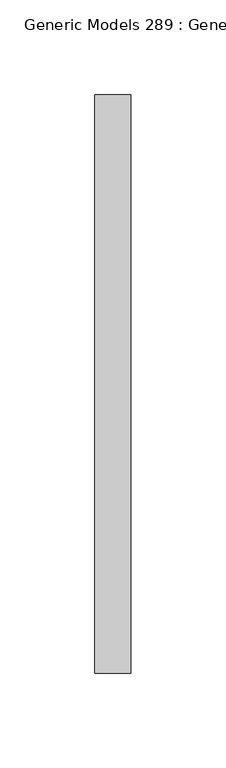
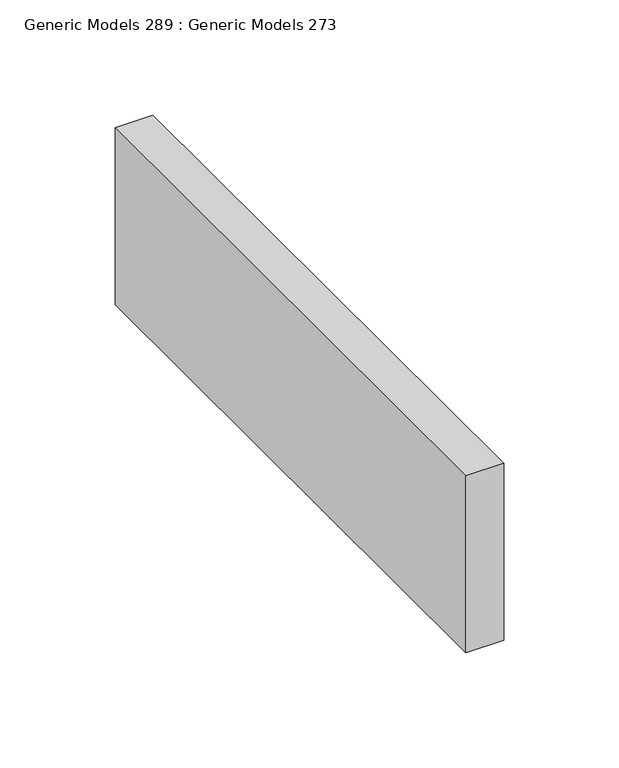
"""IFC4 building model written with IfcOpenShell, lengths in millimetres: proxy geometry, Generic Models 289 : Generic Models 273."""

import ifcopenshell
import ifcopenshell.guid

model = None  # the IFC model being written
_history = None  # IfcOwnerHistory: only IFC2X3 demands one
_inside = {}  # id of a spatial element -> (the spatial element, [elements in it])
_under = {}  # id of a project, library or spatial element -> (it, [spatial elements below it])
_declared = {}  # id of a project -> (the project, [libraries it declares])
_typed = {}  # id of a type object -> (the type object, [elements of that type])
_made_of = {}  # id of a material, layer set ... -> (it, [elements and type objects made of it])


def new_model(schema):
    """Start an empty IFC model of exactly this schema.

    Asked for "IFC4X3", IfcOpenShell would pick the latest addendum, in which some entities
    have other attributes; the version numbers below select the first issue.
    IFC2X3 requires an IfcOwnerHistory on every rooted entity: one is made here for all.
    """
    global model, _history
    if schema == "IFC4X3":
        model = ifcopenshell.file(schema_version=(4, 3, 0, 0))
    else:
        model = ifcopenshell.file(schema=schema)
    _inside.clear()
    _under.clear()
    _declared.clear()
    _typed.clear()
    _made_of.clear()
    _history = None
    if model.schema == "IFC2X3":
        org = make("IfcOrganization", Name="unknown")
        user = make(
            "IfcPersonAndOrganization",
            ThePerson=make("IfcPerson", FamilyName="unknown"),
            TheOrganization=org,
        )
        app = make(
            "IfcApplication",
            ApplicationDeveloper=org,
            Version="unknown",
            ApplicationFullName="unknown",
            ApplicationIdentifier="unknown",
        )
        _history = make(
            "IfcOwnerHistory",
            OwningUser=user,
            OwningApplication=app,
            ChangeAction="ADDED",
            CreationDate=0,
        )
    return model


def make(cls, **values):
    """One entity of the class cls with the attributes given. An attribute that is None is left unset."""
    return model.create_entity(
        cls, **{name: value for name, value in values.items() if value is not None}
    )


def rooted(cls, **values):
    """An entity with a GlobalId (a new one), such as an element, a storey or a relation."""
    return make(cls, GlobalId=ifcopenshell.guid.new(), OwnerHistory=_history, **values)


def si_unit(unit_type, name, prefix=None):
    """IfcSIUnit, for example si_unit("LENGTHUNIT", "METRE", prefix="MILLI")."""
    return make("IfcSIUnit", UnitType=unit_type, Prefix=prefix, Name=name)


def assignment(units):
    """IfcUnitAssignment: the units of a project."""
    return None if units is None else make("IfcUnitAssignment", Units=units)


def point(xyz):
    """IfcCartesianPoint."""
    return None if xyz is None else make("IfcCartesianPoint", Coordinates=xyz)


def direction(xyz):
    """IfcDirection."""
    return None if xyz is None else make("IfcDirection", DirectionRatios=xyz)


def frame(location, z_axis=None, x_axis=None):
    """IfcAxis2Placement3D, a coordinate frame: its origin and axes. An axis left out is left unset."""
    return make(
        "IfcAxis2Placement3D",
        Location=point(location),
        Axis=direction(z_axis),
        RefDirection=direction(x_axis),
    )


def origin():
    """The frame at (0, 0, 0) with its axes left unset."""
    return frame((0.0, 0.0, 0.0))


def place(relative_to, where):
    """IfcLocalPlacement: puts the frame where relative to a parent placement (None: the world)."""
    return make(
        "IfcLocalPlacement", PlacementRelTo=relative_to, RelativePlacement=where
    )


def context(
    kind, dimensions, precision=None, world=None, true_north=None, identifier=None
):
    """IfcGeometricRepresentationContext, for example the 3D "Model" context."""
    return make(
        "IfcGeometricRepresentationContext",
        ContextIdentifier=identifier,
        ContextType=kind,
        CoordinateSpaceDimension=dimensions,
        Precision=precision,
        WorldCoordinateSystem=world,
        TrueNorth=true_north,
    )


def project(units=None, contexts=None):
    """IfcProject with its units and contexts."""
    return rooted(
        "IfcProject",
        Name="project",
        RepresentationContexts=contexts,
        UnitsInContext=assignment(units),
    )


def spatial(cls, under=None, at=None, **own):
    """A site, building, storey or space (cls), placed at a placement, below another one or the project."""
    s = rooted(cls, ObjectPlacement=at, **own)
    if under is not None:
        _under.setdefault(under.id(), (under, []))[1].append(s)
    return s


def polyline(points):
    """IfcPolyline through the points."""
    return make("IfcPolyline", Points=[point(p) for p in points])


def outline(outer, holes=None, kind="AREA"):
    """IfcArbitraryClosedProfileDef: a profile drawn as a closed curve; with holes, ...WithVoids."""
    if holes is None:
        return make("IfcArbitraryClosedProfileDef", ProfileType=kind, OuterCurve=outer)
    return make(
        "IfcArbitraryProfileDefWithVoids",
        ProfileType=kind,
        OuterCurve=outer,
        InnerCurves=holes,
    )


def extrude(swept, where, along, depth):
    """IfcExtrudedAreaSolid: the profile swept, set in the frame where, extruded along a direction by depth."""
    return make(
        "IfcExtrudedAreaSolid",
        SweptArea=swept,
        Position=where,
        ExtrudedDirection=direction(along),
        Depth=depth,
    )


def shape(context_of_items, identifier, shape_type, items):
    """IfcShapeRepresentation: the items that make up one representation, for example the "Body"."""
    return make(
        "IfcShapeRepresentation",
        ContextOfItems=context_of_items,
        RepresentationIdentifier=identifier,
        RepresentationType=shape_type,
        Items=items,
    )


def source(mapping_origin, context_of_items, identifier, shape_type, items):
    """IfcRepresentationMap: a shape defined once, which mapped items show again and again."""
    return make(
        "IfcRepresentationMap",
        MappingOrigin=mapping_origin,
        MappedRepresentation=shape(context_of_items, identifier, shape_type, items),
    )


def transform(
    local_origin,
    x_axis=None,
    y_axis=None,
    z_axis=None,
    scale=None,
    scale2=None,
    scale3=None,
    uniform=True,
):
    """IfcCartesianTransformationOperator3D, or its non-uniform kind. x_axis, y_axis, z_axis: its Axis1, 2, 3."""
    if uniform:
        return make(
            "IfcCartesianTransformationOperator3D",
            Axis1=direction(x_axis),
            Axis2=direction(y_axis),
            LocalOrigin=point(local_origin),
            Scale=scale,
            Axis3=direction(z_axis),
        )
    return make(
        "IfcCartesianTransformationOperator3DnonUniform",
        Axis1=direction(x_axis),
        Axis2=direction(y_axis),
        LocalOrigin=point(local_origin),
        Scale=scale,
        Axis3=direction(z_axis),
        Scale2=scale2,
        Scale3=scale3,
    )


def mapped(mapping_source, mapping_target):
    """IfcMappedItem: shows the shape of a source again, moved by a transform."""
    return make(
        "IfcMappedItem", MappingSource=mapping_source, MappingTarget=mapping_target
    )


def made_of(thing, what):
    """Note that an element or type object is made of a material, layer set ...; save() writes the relation."""
    if what is not None:
        _made_of.setdefault(what.id(), (what, []))[1].append(thing)
    return thing


def element(
    cls,
    number,
    at=None,
    inside=None,
    cuts=None,
    type_object=None,
    material=None,
    context=None,
    identifier="Body",
    shape_type=None,
    held_by="IfcProductDefinitionShape",
    body=None,
    shapes=None,
    **own,
):
    """One element of the class cls, such as IfcWall. Its Tag is "e" and its number.

    at: its placement. inside: the storey or other place that contains it. cuts: it is an
    opening in that element (IfcRelVoidsElement). A single representation is given by context,
    identifier, shape_type and body (its items); several are given by shapes. held_by: the class
    of the entity that holds the representations. save() writes the other relations.
    """
    e = rooted(cls, Tag="e%d" % number, ObjectPlacement=at, **own)
    if body is not None:
        shapes = [shape(context, identifier, shape_type, body)]
    if shapes is not None:
        e.Representation = make(held_by, Representations=shapes)
    if inside is not None:
        _inside.setdefault(inside.id(), (inside, []))[1].append(e)
    if cuts is not None:
        rooted(
            "IfcRelVoidsElement", RelatingBuildingElement=cuts, RelatedOpeningElement=e
        )
    if type_object is not None:
        _typed.setdefault(type_object.id(), (type_object, []))[1].append(e)
    return made_of(e, material)


def aggregate(whole, parts):
    """IfcRelAggregates: a whole, such as a stair, and the parts it consists of."""
    return rooted("IfcRelAggregates", RelatingObject=whole, RelatedObjects=parts)


def save(model, path):
    """Write the relations noted so far, then the file.

    IfcRelAggregates (storeys below a building ...), IfcRelContainedInSpatialStructure (elements
    in a storey), IfcRelDefinesByType, IfcRelAssociatesMaterial and IfcRelDeclares: one each for
    every whole, place, type object, material and project.
    """
    for whole, parts in _under.values():
        aggregate(whole, parts)
    for where, things in _inside.values():
        rooted(
            "IfcRelContainedInSpatialStructure",
            RelatedElements=things,
            RelatingStructure=where,
        )
    for kind, things in _typed.values():
        rooted("IfcRelDefinesByType", RelatedObjects=things, RelatingType=kind)
    for what, things in _made_of.values():
        rooted("IfcRelAssociatesMaterial", RelatedObjects=things, RelatingMaterial=what)
    for by, libraries in _declared.values():
        rooted("IfcRelDeclares", RelatingContext=by, RelatedDefinitions=libraries)
    model.write(path)


def generic_models_289_generic_models_273_24fe49b0(model_context):
    return source(origin(), model_context, "Body", "SweptSolid", [
        extrude(outline(polyline([(1642.0931224, 4564.8872686), (1661.1431224, 4564.8872686), (1661.1431224, 4260.0872686), (1642.0931224, 4260.0872686), (1642.0931224, 4564.8872686)])), frame((0.0, 0.0, 123382.7443431), z_axis=(0.0, 0.0, 1.0), x_axis=(1.0, 0.0, 0.0)), (0.0, 0.0, 1.0), 93.9346579),
    ])


if __name__ == "__main__":
    model = new_model("IFC4")
    model_context = context("Model", 3, world=origin())
    ifc_project = project(units=[si_unit("LENGTHUNIT", "METRE", prefix="MILLI")], contexts=[model_context])
    site = spatial("IfcSite", under=ifc_project)
    building = spatial("IfcBuilding", under=site)
    placement = place(None, origin())
    generic_models_289_generic_models_273_shape = generic_models_289_generic_models_273_24fe49b0(model_context)
    element("IfcBuildingElementProxy", 1, Name="Generic Models 289 : Generic Models 273", ObjectType="Generic Models 289 : Generic Models 273", at=placement, inside=building, context=model_context, shape_type="MappedRepresentation", body=[
        mapped(generic_models_289_generic_models_273_shape, transform((0.0, 0.0, 0.0), x_axis=(1.0, 0.0, 0.0), y_axis=(0.0, 1.0, 0.0), z_axis=(0.0, 0.0, 1.0))),
    ])
    save(model, "model.ifc")

# Revit data of these elements
# Element 1 (IfcBuildingElementProxy, "Generic Models 289 : Generic Models 273")
#   Materials on its faces: "_TREATED BLOCKING AS REQUIRED"
# Materials
#   "_TREATED BLOCKING AS REQUIRED": class "Generic", colour RGB 177 130 114, transparency 0, Cost = 0
